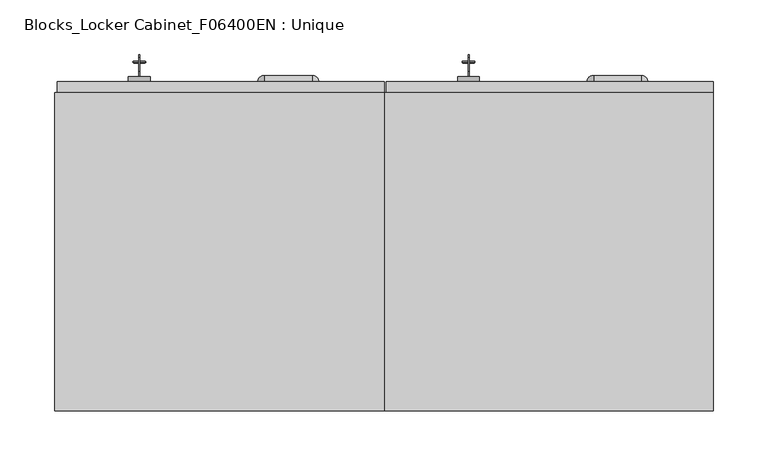
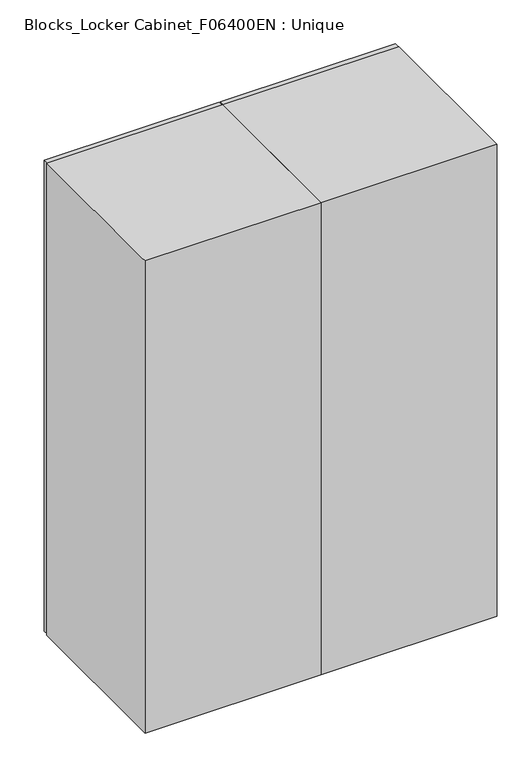
"""IFC4 building model written with IfcOpenShell, lengths in millimetres: furniture geometry, Blocks_Locker Cabinet_F06400EN : Unique."""

from ifc_helpers import new_model, si_unit, point, frame, frame_2d, origin, place, context, project, spatial, polyline, circle_curve, ellipse_curve, trimmed, segment, composite_curve, outline, extrude, faceted_brep, source, transform, mapped, element, save
from ifc_brep_helpers import plane_surface, cylinder_surface, revolved_surface, advanced_brep


def blocks_locker_cabinet_f06400en_unique_75e8493b(model_context):
    return source(origin(), model_context, "Body", "SolidModel", [
        advanced_brep(
        [(-83.0, 12.5, 1375.0), (-63.0, 12.5, 1375.0), (-71.1588195, 12.5, 1382.0962926), (-74.8411805, 12.5, 1382.0962926), (-74.8411805, 12.5, 1372.8618188), (-71.1588195, 12.5, 1372.8618188), (-83.0, 7.5, 1375.0), (-63.0, 7.5, 1375.0), (-63.0, 10.7450625, 1375.0), (-83.0, 10.7450625, 1375.0), (-71.1588195, 10.7450625, 1372.8618188), (-71.1588195, 10.7450625, 1382.0962926), (-74.8411805, 10.7450625, 1372.8618188), (-74.8411805, 10.7450625, 1382.0962926)],
        [
            (0, 1, circle_curve(frame((-73.0, 12.5, 1375.0), z_axis=(0.0, 1.0, 0.0), x_axis=(1.0, 0.0, 0.0)), 10.0)),
            (1, 0, circle_curve(frame((-73.0, 12.5, 1375.0), z_axis=(0.0, 1.0, 0.0), x_axis=(1.0, 0.0, 0.0)), 10.0)),
            (2, 3),
            (3, 4),
            (4, 5),
            (5, 2),
            (6, 7, circle_curve(frame((-73.0, 7.5, 1375.0), z_axis=(0.0, -1.0, 0.0), x_axis=(1.0, 0.0, 0.0)), 10.0)),
            (7, 6, circle_curve(frame((-73.0, 7.5, 1375.0), z_axis=(0.0, -1.0, 0.0), x_axis=(1.0, 0.0, 0.0)), 10.0)),
            (1, 8),
            (8, 7),
            (6, 9),
            (9, 0),
            (5, 10),
            (10, 11),
            (11, 2),
            (4, 12),
            (12, 10),
            (3, 13),
            (13, 12),
            (11, 13),
        ],
        [
            plane_surface(frame((-63.0, 12.5, 1375.0), z_axis=(0.0, 1.0, 0.0), x_axis=(0.0, 0.0, 1.0))),
            plane_surface(frame((-63.0, 7.5, 1375.0), z_axis=(0.0, -1.0, 0.0), x_axis=(0.0, 0.0, -1.0))),
            cylinder_surface(frame((-73.0, 7.5, 1375.0), z_axis=(0.0, 1.0, 0.0), x_axis=(1.0, 0.0, 0.0)), 10.0),
            plane_surface(frame((-71.1588195, 12.5, 1382.0962926), z_axis=(-1.0, 0.0, 0.0), x_axis=(0.0, -1.0, 0.0))),
            plane_surface(frame((-71.1588195, 12.5, 1372.8618188), z_axis=(0.0, 0.0, 1.0), x_axis=(0.0, -1.0, 0.0))),
            plane_surface(frame((-74.8411805, 12.5, 1372.8618188), z_axis=(1.0, 0.0, 0.0), x_axis=(0.0, -1.0, 0.0))),
            plane_surface(frame((-74.8411805, 12.5, 1382.0962926), z_axis=(0.0, 0.0, -1.0), x_axis=(0.0, -1.0, 0.0))),
            plane_surface(frame((-63.0, 10.7450625, 1375.0), z_axis=(0.0, 1.0, 0.0), x_axis=(0.0, 0.0, 1.0))),
        ],
        [
            (0, [[1, 2], [3, 4, 5, 6]]),
            (1, [[7, 8]]),
            (2, [[9, 10, -7, 11, 12, -2]]),
            (2, [[-12, -11, -8, -10, -9, -1]]),
            (3, [[13, 14, 15, -6]]),
            (4, [[16, 17, -13, -5]]),
            (5, [[18, 19, -16, -4]]),
            (6, [[-15, 20, -18, -3]]),
            (7, [[-17, -19, -20, -14]]),
        ],
    ),
        extrude(outline(composite_curve([segment(polyline([(16.8246351, 1372.8618188), (13.7848488, 1372.8618188)]), True, "CONTINUOUS"), segment(trimmed(circle_curve(frame_2d((12.908516, 1372.8618188)), 0.8763328), [point((13.7848488, 1372.8618188))], [point((12.0321832, 1372.8618188))], True, "CARTESIAN"), True, "CONTINUOUS"), segment(polyline([(12.0321832, 1372.8618188), (10.7450625, 1372.8618188), (10.7450625, 1377.6669902), (17.0336838, 1377.6669902)]), True, "CONTINUOUS"), segment(trimmed(circle_curve(frame_2d((23.0067332, 1375.0)), 6.5414185), [point((17.0336838, 1377.6669902))], [point((16.8246351, 1372.8618188))], False, "CARTESIAN"), True, "CONTINUOUS")], self_intersect=False), holes=[composite_curve([segment(trimmed(circle_curve(frame_2d((25.6281997, 1375.0)), 1.688217), [point((27.3164167, 1375.0))], [point((23.9399827, 1375.0))], True, "CARTESIAN"), True, "CONTINUOUS"), segment(trimmed(circle_curve(frame_2d((25.6281997, 1375.0)), 1.688217), [point((23.9399827, 1375.0))], [point((27.3164167, 1375.0))], True, "CARTESIAN"), True, "CONTINUOUS")], self_intersect=False)]), frame((-73.4043078, 0.0, 0.0), z_axis=(1.0, 0.0, 0.0), x_axis=(0.0, 1.0, 0.0)), (0.0, 0.0, 1.0), 0.9157402),
        extrude(outline(composite_curve([segment(polyline([(27.8125, 1354.8018875), (27.8125, 1351.7621012)]), True, "CONTINUOUS"), segment(trimmed(circle_curve(frame_2d((27.8125, 1350.8857684)), 0.8763328), [point((27.8125, 1351.7621012))], [point((27.8125, 1350.0094356))], True, "CARTESIAN"), True, "CONTINUOUS"), segment(polyline([(27.8125, 1350.0094356), (27.8125, 1347.7621012)]), True, "CONTINUOUS"), segment(trimmed(circle_curve(frame_2d((27.8125, 1346.8857684)), 0.8763328), [point((27.8125, 1347.7621012))], [point((27.8125, 1346.0094356))], True, "CARTESIAN"), True, "CONTINUOUS"), segment(polyline([(27.8125, 1346.0094356), (27.8125, 1343.7621012)]), True, "CONTINUOUS"), segment(trimmed(circle_curve(frame_2d((27.8125, 1342.8857684)), 0.8763328), [point((27.8125, 1343.7621012))], [point((27.8125, 1342.0094356))], True, "CARTESIAN"), True, "CONTINUOUS"), segment(polyline([(27.8125, 1342.0094356), (27.8125, 1340.3532579), (25.9613419, 1337.7095301), (24.2573286, 1337.7095301), (24.2573286, 1354.5978839)]), True, "CONTINUOUS"), segment(trimmed(circle_curve(frame_2d((25.6743188, 1360.9839856)), 6.5414185), [point((24.2573286, 1354.5978839))], [point((27.8125, 1354.8018875))], False, "CARTESIAN"), True, "CONTINUOUS")], self_intersect=False), holes=[composite_curve([segment(trimmed(circle_curve(frame_2d((25.6743188, 1363.6054521)), 1.688217), [point((25.6743188, 1365.2936691))], [point((25.6743188, 1361.9172351))], True, "CARTESIAN"), True, "CONTINUOUS"), segment(trimmed(circle_curve(frame_2d((25.6743188, 1363.6054521)), 1.688217), [point((25.6743188, 1361.9172351))], [point((25.6743188, 1365.2936691))], True, "CARTESIAN"), True, "CONTINUOUS")], self_intersect=False)]), frame((-73.4043078, 0.0, 0.0), z_axis=(1.0, 0.0, 0.0), x_axis=(0.0, 1.0, 0.0)), (0.0, 0.0, 1.0), 0.9157402),
        advanced_brep(
        [(-68.8, 25.663019, 1369.4000012), (-67.2, 25.663019, 1369.4000012), (-78.8, 25.663019, 1369.4000012), (-77.2, 25.663019, 1369.4000012)],
        [
            (0, 1, circle_curve(frame((-68.0, 25.663019, 1369.4000012), z_axis=(0.0, 0.0, -1.0), x_axis=(-1.0, 0.0, 0.0)), 0.8)),
            (1, 2, circle_curve(frame((-73.0, 25.663019, 1369.4000012), z_axis=(0.0, 1.0, 0.0), x_axis=(-1.0, 0.0, 0.0)), 5.8)),
            (2, 3, circle_curve(frame((-78.0, 25.663019, 1369.4000012), z_axis=(0.0, 0.0, -1.0), x_axis=(1.0, 0.0, 0.0)), 0.8)),
            (3, 0, circle_curve(frame((-73.0, 25.663019, 1369.4000012), z_axis=(0.0, -1.0, 0.0), x_axis=(-1.0, 0.0, 0.0)), 4.2)),
            (1, 0, circle_curve(frame((-68.0, 25.663019, 1369.4000012), z_axis=(0.0, 0.0, -1.0), x_axis=(-1.0, 0.0, 0.0)), 0.8)),
            (3, 2, circle_curve(frame((-78.0, 25.663019, 1369.4000012), z_axis=(0.0, 0.0, -1.0), x_axis=(1.0, 0.0, 0.0)), 0.8)),
            (2, 1, circle_curve(frame((-73.0, 25.663019, 1369.4000012), z_axis=(0.0, 1.0, 0.0), x_axis=(1.0, 0.0, 0.0)), 5.8)),
            (0, 3, circle_curve(frame((-73.0, 25.663019, 1369.4000012), z_axis=(0.0, -1.0, 0.0), x_axis=(1.0, 0.0, 0.0)), 4.2)),
        ],
        [
            revolved_surface(trimmed(ellipse_curve(frame((-78.0, 25.663019, 1369.4000012), z_axis=(0.0, 0.0, -1.0), x_axis=(1.0, 0.0, 0.0)), 0.8, 0.8), [point((-78.8, 25.663019, 1369.4000012))], [point((-77.2, 25.663019, 1369.4000012))], True, "CARTESIAN"), (-73.0, -2.5, 1369.4000012), (0.0, 1.0, 0.0)),
            revolved_surface(trimmed(ellipse_curve(frame((-78.0, 25.663019, 1369.4000012), z_axis=(0.0, 0.0, -1.0), x_axis=(1.0, 0.0, 0.0)), 0.8, 0.8), [point((-77.2, 25.663019, 1369.4000012))], [point((-78.8, 25.663019, 1369.4000012))], True, "CARTESIAN"), (-73.0, -2.5, 1369.4000012), (0.0, 1.0, 0.0)),
            revolved_surface(trimmed(ellipse_curve(frame((-68.0, 25.663019, 1369.4000012), z_axis=(0.0, 0.0, 1.0), x_axis=(-1.0, 0.0, 0.0)), 0.8, 0.8), [point((-67.2, 25.663019, 1369.4000012))], [point((-68.8, 25.663019, 1369.4000012))], True, "CARTESIAN"), (-73.0, -2.5, 1369.4000012), (0.0, 1.0, 0.0)),
            revolved_surface(trimmed(ellipse_curve(frame((-68.0, 25.663019, 1369.4000012), z_axis=(0.0, 0.0, 1.0), x_axis=(-1.0, 0.0, 0.0)), 0.8, 0.8), [point((-68.8, 25.663019, 1369.4000012))], [point((-67.2, 25.663019, 1369.4000012))], True, "CARTESIAN"), (-73.0, -2.5, 1369.4000012), (0.0, 1.0, 0.0)),
        ],
        [
            (0, [[1, 2, 3, 4]]),
            (1, [[5, -4, 6, -2]]),
            (2, [[-3, 7, -1, 8]]),
            (3, [[-6, -8, -5, -7]]),
        ],
    ),
        advanced_brep(
        [(-148.0, 7.5, 1799.0), (-148.0, -2.5, 1799.0), (150.0, -2.5, 1799.0), (150.0, 7.5, 1799.0), (-148.0, 7.5, 951.0), (150.0, 7.5, 951.0), (150.0, -2.5, 951.0), (-148.0, -2.5, 951.0), (-93.0, 7.5, 1525.0), (-93.0, 7.5, 1405.0), (-33.7890736, 7.5, 1405.0), (-33.7890736, 7.5, 1525.0), (-80.6526901, 0.3712773, 1525.0), (-57.2105549, 3.975278, 1525.0), (-80.6526901, 0.3712773, 1405.0), (-57.2105549, 3.975278, 1405.0)],
        [
            (0, 1),
            (1, 2),
            (2, 3),
            (3, 0),
            (4, 5),
            (5, 6),
            (6, 7),
            (7, 4),
            (3, 5),
            (4, 0),
            (8, 9),
            (9, 10),
            (10, 11),
            (11, 8),
            (2, 6),
            (1, 7),
            (12, 8),
            (11, 13),
            (13, 12, circle_curve(frame((-71.1776523, 16.7825242, 1525.0), z_axis=(0.0, 0.0, -1.0), x_axis=(0.0, 1.0, 0.0)), 18.9500756)),
            (14, 15, circle_curve(frame((-71.1776523, 16.7825242, 1405.0), z_axis=(0.0, 0.0, 1.0), x_axis=(0.0, 1.0, 0.0)), 18.9500756)),
            (15, 10),
            (9, 14),
            (12, 14),
            (15, 13),
        ],
        [
            plane_surface(frame((150.0, 7.5, 1799.0), z_axis=(0.0, 0.0, 1.0), x_axis=(1.0, 0.0, 0.0))),
            plane_surface(frame((150.0, 7.5, 951.0), z_axis=(0.0, 0.0, -1.0), x_axis=(-1.0, 0.0, 0.0))),
            plane_surface(frame((-148.0, 7.5, 1799.0), z_axis=(0.0, 1.0, 0.0), x_axis=(0.0, 0.0, -1.0))),
            plane_surface(frame((150.0, 7.5, 1799.0), z_axis=(1.0, 0.0, 0.0), x_axis=(0.0, 0.0, -1.0))),
            plane_surface(frame((150.0, -2.5, 1799.0), z_axis=(0.0, -1.0, 0.0), x_axis=(0.0, 0.0, -1.0))),
            plane_surface(frame((-148.0, -2.5, 1799.0), z_axis=(-1.0, 0.0, 0.0), x_axis=(0.0, 0.0, -1.0))),
            plane_surface(frame((-93.0, 7.5, 1525.0), z_axis=(0.0, 0.0, -1.0), x_axis=(-0.866025403784437, 0.5000000000000028, 0.0))),
            plane_surface(frame((-93.0, 7.5, 1405.0), z_axis=(0.0, 0.0, 1.0), x_axis=(0.866025403784437, -0.5000000000000028, 0.0))),
            plane_surface(frame((-80.6526901, 0.3712773, 1525.0), z_axis=(0.5000000000000028, 0.866025403784437, 0.0), x_axis=(0.0, 0.0, -1.0))),
            plane_surface(frame((-33.7890736, 7.5, 1525.0), z_axis=(-0.14881527984319862, 0.9888650122666847, 0.0), x_axis=(0.0, 0.0, -1.0))),
            revolved_surface(polyline([(-71.1776523, 35.7325998, 1525.0), (-71.1776523, 35.7325998, 1405.0)]), (-71.1776523, 16.7825242, 1405.0), (0.0, 0.0, 1.0)),
        ],
        [
            (0, [[1, 2, 3, 4]]),
            (1, [[5, 6, 7, 8]]),
            (2, [[9, -5, 10, -4], [11, 12, 13, 14]]),
            (3, [[15, -6, -9, -3]]),
            (4, [[16, -7, -15, -2]]),
            (5, [[-10, -8, -16, -1]]),
            (6, [[17, -14, 18, 19]]),
            (7, [[20, 21, -12, 22]]),
            (8, [[23, -22, -11, -17]]),
            (9, [[-13, -21, 24, -18]]),
            (10, [[-24, -20, -23, -19]]),
        ],
    ),
        advanced_brep(
        [(35.0, 7.5, 991.0), (90.5189667, 7.5, 991.0), (84.5189667, 7.5, 997.0), (41.0, 7.5, 997.0), (41.0, 13.5, 991.0), (84.5189667, 13.5, 991.0)],
        [
            (0, 1),
            (1, 2, circle_curve(frame((84.5189667, 7.5, 991.0), z_axis=(0.0, -1.0, 0.0), x_axis=(1.0, 0.0, 0.0)), 6.0)),
            (2, 3),
            (3, 0, circle_curve(frame((41.0, 7.5, 991.0), z_axis=(0.0, -1.0, 0.0), x_axis=(1.0, 0.0, 0.0)), 6.0)),
            (0, 4, circle_curve(frame((41.0, 7.5, 991.0), z_axis=(0.0, 0.0, -1.0), x_axis=(1.0, 0.0, 0.0)), 6.0)),
            (4, 5),
            (5, 1, circle_curve(frame((84.5189667, 7.5, 991.0), z_axis=(0.0, 0.0, -1.0), x_axis=(1.0, 0.0, 0.0)), 6.0)),
            (3, 4, circle_curve(frame((41.0, 7.5, 991.0), z_axis=(-1.0, 0.0, 0.0), x_axis=(0.0, 0.0, 1.0)), 6.0)),
            (2, 5, circle_curve(frame((84.5189667, 7.5, 991.0), z_axis=(-1.0, 0.0, 0.0), x_axis=(0.0, 0.0, 1.0)), 6.0)),
        ],
        [
            plane_surface(frame((85.0, 7.5, 991.0), z_axis=(0.0, -1.0, 0.0), x_axis=(0.0, 0.0, 1.0))),
            plane_surface(frame((85.0, 7.5, 991.0), z_axis=(0.0, 0.0, -1.0), x_axis=(0.0, 1.0, 0.0))),
            revolved_surface(trimmed(ellipse_curve(frame((41.0, 7.5, 991.0), z_axis=(0.0, 1.0, 0.0), x_axis=(1.0, 0.0, 0.0)), 6.0, 6.0), [point((35.0, 7.5, 991.0))], [point((41.0, 7.5, 997.0))], True, "CARTESIAN"), (85.0, 7.5, 991.0), (1.0, 0.0, 0.0)),
            cylinder_surface(frame((85.0, 7.5, 991.0), z_axis=(1.0, 0.0, 0.0), x_axis=(0.0, 0.0, 1.0)), 6.0),
            revolved_surface(trimmed(ellipse_curve(frame((84.5189667, 7.5, 991.0), z_axis=(0.0, 1.0, 0.0), x_axis=(1.0, 0.0, 0.0)), 6.0, 6.0), [point((84.5189667, 7.5, 997.0))], [point((90.5189667, 7.5, 991.0))], True, "CARTESIAN"), (85.0, 7.5, 991.0), (1.0, 0.0, 0.0)),
        ],
        [
            (0, [[1, 2, 3, 4]]),
            (1, [[-1, 5, 6, 7]]),
            (2, [[-5, -4, 8]]),
            (3, [[-6, -8, -3, 9]]),
            (4, [[-7, -9, -2]]),
        ],
    ),
        advanced_brep(
        [(35.0, 7.5, 1006.0), (90.5189667, 7.5, 1006.0), (84.5189667, 7.5, 1012.0), (41.0, 7.5, 1012.0), (41.0, 13.5, 1006.0), (84.5189667, 13.5, 1006.0)],
        [
            (0, 1),
            (1, 2, circle_curve(frame((84.5189667, 7.5, 1006.0), z_axis=(0.0, -1.0, 0.0), x_axis=(1.0, 0.0, 0.0)), 6.0)),
            (2, 3),
            (3, 0, circle_curve(frame((41.0, 7.5, 1006.0), z_axis=(0.0, -1.0, 0.0), x_axis=(1.0, 0.0, 0.0)), 6.0)),
            (0, 4, circle_curve(frame((41.0, 7.5, 1006.0), z_axis=(0.0, 0.0, -1.0), x_axis=(1.0, 0.0, 0.0)), 6.0)),
            (4, 5),
            (5, 1, circle_curve(frame((84.5189667, 7.5, 1006.0), z_axis=(0.0, 0.0, -1.0), x_axis=(1.0, 0.0, 0.0)), 6.0)),
            (3, 4, circle_curve(frame((41.0, 7.5, 1006.0), z_axis=(-1.0, 0.0, 0.0), x_axis=(0.0, 0.0, 1.0)), 6.0)),
            (2, 5, circle_curve(frame((84.5189667, 7.5, 1006.0), z_axis=(-1.0, 0.0, 0.0), x_axis=(0.0, 0.0, 1.0)), 6.0)),
        ],
        [
            plane_surface(frame((85.0, 7.5, 1006.0), z_axis=(0.0, -1.0, 0.0), x_axis=(0.0, 0.0, 1.0))),
            plane_surface(frame((85.0, 7.5, 1006.0), z_axis=(0.0, 0.0, -1.0), x_axis=(0.0, 1.0, 0.0))),
            revolved_surface(trimmed(ellipse_curve(frame((41.0, 7.5, 1006.0), z_axis=(0.0, 1.0, 0.0), x_axis=(1.0, 0.0, 0.0)), 6.0, 6.0), [point((35.0, 7.5, 1006.0))], [point((41.0, 7.5, 1012.0))], True, "CARTESIAN"), (85.0, 7.5, 1006.0), (1.0, 0.0, 0.0)),
            cylinder_surface(frame((85.0, 7.5, 1006.0), z_axis=(1.0, 0.0, 0.0), x_axis=(0.0, 0.0, 1.0)), 6.0),
            revolved_surface(trimmed(ellipse_curve(frame((84.5189667, 7.5, 1006.0), z_axis=(0.0, 1.0, 0.0), x_axis=(1.0, 0.0, 0.0)), 6.0, 6.0), [point((84.5189667, 7.5, 1012.0))], [point((90.5189667, 7.5, 1006.0))], True, "CARTESIAN"), (85.0, 7.5, 1006.0), (1.0, 0.0, 0.0)),
        ],
        [
            (0, [[1, 2, 3, 4]]),
            (1, [[-1, 5, 6, 7]]),
            (2, [[-5, -4, 8]]),
            (3, [[-6, -8, -3, 9]]),
            (4, [[-7, -9, -2]]),
        ],
    ),
        advanced_brep(
        [(35.0, 7.5, 1021.0), (90.5189667, 7.5, 1021.0), (84.5189667, 7.5, 1027.0), (41.0, 7.5, 1027.0), (41.0, 13.5, 1021.0), (84.5189667, 13.5, 1021.0)],
        [
            (0, 1),
            (1, 2, circle_curve(frame((84.5189667, 7.5, 1021.0), z_axis=(0.0, -1.0, 0.0), x_axis=(1.0, 0.0, 0.0)), 6.0)),
            (2, 3),
            (3, 0, circle_curve(frame((41.0, 7.5, 1021.0), z_axis=(0.0, -1.0, 0.0), x_axis=(1.0, 0.0, 0.0)), 6.0)),
            (0, 4, circle_curve(frame((41.0, 7.5, 1021.0), z_axis=(0.0, 0.0, -1.0), x_axis=(1.0, 0.0, 0.0)), 6.0)),
            (4, 5),
            (5, 1, circle_curve(frame((84.5189667, 7.5, 1021.0), z_axis=(0.0, 0.0, -1.0), x_axis=(1.0, 0.0, 0.0)), 6.0)),
            (3, 4, circle_curve(frame((41.0, 7.5, 1021.0), z_axis=(-1.0, 0.0, 0.0), x_axis=(0.0, 0.0, 1.0)), 6.0)),
            (2, 5, circle_curve(frame((84.5189667, 7.5, 1021.0), z_axis=(-1.0, 0.0, 0.0), x_axis=(0.0, 0.0, 1.0)), 6.0)),
        ],
        [
            plane_surface(frame((85.0, 7.5, 1021.0), z_axis=(0.0, -1.0, 0.0), x_axis=(0.0, 0.0, 1.0))),
            plane_surface(frame((85.0, 7.5, 1021.0), z_axis=(0.0, 0.0, -1.0), x_axis=(0.0, 1.0, 0.0))),
            revolved_surface(trimmed(ellipse_curve(frame((41.0, 7.5, 1021.0), z_axis=(0.0, 1.0, 0.0), x_axis=(1.0, 0.0, 0.0)), 6.0, 6.0), [point((35.0, 7.5, 1021.0))], [point((41.0, 7.5, 1027.0))], True, "CARTESIAN"), (85.0, 7.5, 1021.0), (1.0, 0.0, 0.0)),
            cylinder_surface(frame((85.0, 7.5, 1021.0), z_axis=(1.0, 0.0, 0.0), x_axis=(0.0, 0.0, 1.0)), 6.0),
            revolved_surface(trimmed(ellipse_curve(frame((84.5189667, 7.5, 1021.0), z_axis=(0.0, 1.0, 0.0), x_axis=(1.0, 0.0, 0.0)), 6.0, 6.0), [point((84.5189667, 7.5, 1027.0))], [point((90.5189667, 7.5, 1021.0))], True, "CARTESIAN"), (85.0, 7.5, 1021.0), (1.0, 0.0, 0.0)),
        ],
        [
            (0, [[1, 2, 3, 4]]),
            (1, [[-1, 5, 6, 7]]),
            (2, [[-5, -4, 8]]),
            (3, [[-6, -8, -3, 9]]),
            (4, [[-7, -9, -2]]),
        ],
    ),
        advanced_brep(
        [(35.0, 7.5, 1036.0), (90.5189667, 7.5, 1036.0), (84.5189667, 7.5, 1042.0), (41.0, 7.5, 1042.0), (41.0, 13.5, 1036.0), (84.5189667, 13.5, 1036.0)],
        [
            (0, 1),
            (1, 2, circle_curve(frame((84.5189667, 7.5, 1036.0), z_axis=(0.0, -1.0, 0.0), x_axis=(1.0, 0.0, 0.0)), 6.0)),
            (2, 3),
            (3, 0, circle_curve(frame((41.0, 7.5, 1036.0), z_axis=(0.0, -1.0, 0.0), x_axis=(1.0, 0.0, 0.0)), 6.0)),
            (0, 4, circle_curve(frame((41.0, 7.5, 1036.0), z_axis=(0.0, 0.0, -1.0), x_axis=(1.0, 0.0, 0.0)), 6.0)),
            (4, 5),
            (5, 1, circle_curve(frame((84.5189667, 7.5, 1036.0), z_axis=(0.0, 0.0, -1.0), x_axis=(1.0, 0.0, 0.0)), 6.0)),
            (3, 4, circle_curve(frame((41.0, 7.5, 1036.0), z_axis=(-1.0, 0.0, 0.0), x_axis=(0.0, 0.0, 1.0)), 6.0)),
            (2, 5, circle_curve(frame((84.5189667, 7.5, 1036.0), z_axis=(-1.0, 0.0, 0.0), x_axis=(0.0, 0.0, 1.0)), 6.0)),
        ],
        [
            plane_surface(frame((85.0, 7.5, 1036.0), z_axis=(0.0, -1.0, 0.0), x_axis=(0.0, 0.0, 1.0))),
            plane_surface(frame((85.0, 7.5, 1036.0), z_axis=(0.0, 0.0, -1.0), x_axis=(0.0, 1.0, 0.0))),
            revolved_surface(trimmed(ellipse_curve(frame((41.0, 7.5, 1036.0), z_axis=(0.0, 1.0, 0.0), x_axis=(1.0, 0.0, 0.0)), 6.0, 6.0), [point((35.0, 7.5, 1036.0))], [point((41.0, 7.5, 1042.0))], True, "CARTESIAN"), (85.0, 7.5, 1036.0), (1.0, 0.0, 0.0)),
            cylinder_surface(frame((85.0, 7.5, 1036.0), z_axis=(1.0, 0.0, 0.0), x_axis=(0.0, 0.0, 1.0)), 6.0),
            revolved_surface(trimmed(ellipse_curve(frame((84.5189667, 7.5, 1036.0), z_axis=(0.0, 1.0, 0.0), x_axis=(1.0, 0.0, 0.0)), 6.0, 6.0), [point((84.5189667, 7.5, 1042.0))], [point((90.5189667, 7.5, 1036.0))], True, "CARTESIAN"), (85.0, 7.5, 1036.0), (1.0, 0.0, 0.0)),
        ],
        [
            (0, [[1, 2, 3, 4]]),
            (1, [[-1, 5, 6, 7]]),
            (2, [[-5, -4, 8]]),
            (3, [[-6, -8, -3, 9]]),
            (4, [[-7, -9, -2]]),
        ],
    ),
        advanced_brep(
        [(35.0, 7.5, 1051.0), (90.5189667, 7.5, 1051.0), (84.5189667, 7.5, 1057.0), (41.0, 7.5, 1057.0), (41.0, 13.5, 1051.0), (84.5189667, 13.5, 1051.0)],
        [
            (0, 1),
            (1, 2, circle_curve(frame((84.5189667, 7.5, 1051.0), z_axis=(0.0, -1.0, 0.0), x_axis=(1.0, 0.0, 0.0)), 6.0)),
            (2, 3),
            (3, 0, circle_curve(frame((41.0, 7.5, 1051.0), z_axis=(0.0, -1.0, 0.0), x_axis=(1.0, 0.0, 0.0)), 6.0)),
            (0, 4, circle_curve(frame((41.0, 7.5, 1051.0), z_axis=(0.0, 0.0, -1.0), x_axis=(1.0, 0.0, 0.0)), 6.0)),
            (4, 5),
            (5, 1, circle_curve(frame((84.5189667, 7.5, 1051.0), z_axis=(0.0, 0.0, -1.0), x_axis=(1.0, 0.0, 0.0)), 6.0)),
            (3, 4, circle_curve(frame((41.0, 7.5, 1051.0), z_axis=(-1.0, 0.0, 0.0), x_axis=(0.0, 0.0, 1.0)), 6.0)),
            (2, 5, circle_curve(frame((84.5189667, 7.5, 1051.0), z_axis=(-1.0, 0.0, 0.0), x_axis=(0.0, 0.0, 1.0)), 6.0)),
        ],
        [
            plane_surface(frame((85.0, 7.5, 1051.0), z_axis=(0.0, -1.0, 0.0), x_axis=(0.0, 0.0, 1.0))),
            plane_surface(frame((85.0, 7.5, 1051.0), z_axis=(0.0, 0.0, -1.0), x_axis=(0.0, 1.0, 0.0))),
            revolved_surface(trimmed(ellipse_curve(frame((41.0, 7.5, 1051.0), z_axis=(0.0, 1.0, 0.0), x_axis=(1.0, 0.0, 0.0)), 6.0, 6.0), [point((35.0, 7.5, 1051.0))], [point((41.0, 7.5, 1057.0))], True, "CARTESIAN"), (85.0, 7.5, 1051.0), (1.0, 0.0, 0.0)),
            cylinder_surface(frame((85.0, 7.5, 1051.0), z_axis=(1.0, 0.0, 0.0), x_axis=(0.0, 0.0, 1.0)), 6.0),
            revolved_surface(trimmed(ellipse_curve(frame((84.5189667, 7.5, 1051.0), z_axis=(0.0, 1.0, 0.0), x_axis=(1.0, 0.0, 0.0)), 6.0, 6.0), [point((84.5189667, 7.5, 1057.0))], [point((90.5189667, 7.5, 1051.0))], True, "CARTESIAN"), (85.0, 7.5, 1051.0), (1.0, 0.0, 0.0)),
        ],
        [
            (0, [[1, 2, 3, 4]]),
            (1, [[-1, 5, 6, 7]]),
            (2, [[-5, -4, 8]]),
            (3, [[-6, -8, -3, 9]]),
            (4, [[-7, -9, -2]]),
        ],
    ),
        extrude(outline(composite_curve([segment(polyline([(-80.6526901, 0.3712773), (-93.0, 7.5), (-33.7890736, 7.5), (-57.2105549, 3.975278)]), True, "CONTINUOUS"), segment(trimmed(circle_curve(frame_2d((-71.1776523, 16.7825242)), 18.9500756), [point((-57.2105549, 3.975278))], [point((-80.6526901, 0.3712773))], False, "CARTESIAN"), True, "CONTINUOUS")], self_intersect=False)), frame((0.0, 0.0, 1405.0), z_axis=(0.0, 0.0, 1.0), x_axis=(1.0, 0.0, 0.0)), (0.0, 0.0, 1.0), 5.0),
        extrude(outline(composite_curve([segment(polyline([(-80.6526901, 0.3712773), (-93.0, 7.5), (-33.7890736, 7.5), (-57.2105549, 3.975278)]), True, "CONTINUOUS"), segment(trimmed(circle_curve(frame_2d((-71.1776523, 16.7825242)), 18.9500756), [point((-57.2105549, 3.975278))], [point((-80.6526901, 0.3712773))], False, "CARTESIAN"), True, "CONTINUOUS")], self_intersect=False)), frame((0.0, 0.0, 1520.0), z_axis=(0.0, 0.0, 1.0), x_axis=(1.0, 0.0, 0.0)), (0.0, 0.0, 1.0), 5.0),
        faceted_brep([(150.0, -2.5, 1800.0), (150.0, -2.5, 950.0), (-150.0, -2.5, 950.0), (-150.0, -2.5, 1800.0), (140.0, -2.5, 1790.0), (-140.0, -2.5, 1790.0), (-140.0, -2.5, 960.0), (140.0, -2.5, 960.0), (150.0, -292.5, 1800.0), (-150.0, -292.5, 1800.0), (-150.0, -292.5, 950.0), (150.0, -292.5, 950.0), (-150.0, -282.5, 1800.0), (150.0, -282.5, 1800.0), (-150.0, -282.5, 950.0), (150.0, -282.5, 950.0), (140.0, -282.5, 960.0), (140.0, -282.5, 1790.0), (-140.0, -282.5, 960.0), (-140.0, -282.5, 1790.0)], [[[0, 1, 2, 3], [4, 5, 6, 7]], [[8, 9, 10, 11]], [[3, 12, 9, 8, 13, 0]], [[2, 14, 10, 9, 12, 3]], [[1, 15, 11, 10, 14, 2]], [[0, 13, 8, 11, 15, 1]], [[7, 16, 17, 4]], [[6, 18, 16, 7]], [[5, 19, 18, 6]], [[4, 17, 19, 5]], [[16, 18, 19, 17]]]),
        advanced_brep(
        [(217.0, 12.5, 1375.0), (237.0, 12.5, 1375.0), (228.8411805, 12.5, 1382.0962926), (225.1588195, 12.5, 1382.0962926), (225.1588195, 12.5, 1372.8618188), (228.8411805, 12.5, 1372.8618188), (217.0, 7.5, 1375.0), (237.0, 7.5, 1375.0), (237.0, 10.7450625, 1375.0), (217.0, 10.7450625, 1375.0), (228.8411805, 10.7450625, 1372.8618188), (228.8411805, 10.7450625, 1382.0962926), (225.1588195, 10.7450625, 1372.8618188), (225.1588195, 10.7450625, 1382.0962926)],
        [
            (0, 1, circle_curve(frame((227.0, 12.5, 1375.0), z_axis=(0.0, 1.0, 0.0), x_axis=(1.0, 0.0, 0.0)), 10.0)),
            (1, 0, circle_curve(frame((227.0, 12.5, 1375.0), z_axis=(0.0, 1.0, 0.0), x_axis=(1.0, 0.0, 0.0)), 10.0)),
            (2, 3),
            (3, 4),
            (4, 5),
            (5, 2),
            (6, 7, circle_curve(frame((227.0, 7.5, 1375.0), z_axis=(0.0, -1.0, 0.0), x_axis=(1.0, 0.0, 0.0)), 10.0)),
            (7, 6, circle_curve(frame((227.0, 7.5, 1375.0), z_axis=(0.0, -1.0, 0.0), x_axis=(1.0, 0.0, 0.0)), 10.0)),
            (1, 8),
            (8, 7),
            (6, 9),
            (9, 0),
            (5, 10),
            (10, 11),
            (11, 2),
            (4, 12),
            (12, 10),
            (3, 13),
            (13, 12),
            (11, 13),
        ],
        [
            plane_surface(frame((237.0, 12.5, 1375.0), z_axis=(0.0, 1.0, 0.0), x_axis=(0.0, 0.0, 1.0))),
            plane_surface(frame((237.0, 7.5, 1375.0), z_axis=(0.0, -1.0, 0.0), x_axis=(0.0, 0.0, -1.0))),
            cylinder_surface(frame((227.0, 7.5, 1375.0), z_axis=(0.0, 1.0, 0.0), x_axis=(1.0, 0.0, 0.0)), 10.0),
            plane_surface(frame((228.8411805, 12.5, 1382.0962926), z_axis=(-1.0, 0.0, 0.0), x_axis=(0.0, -1.0, 0.0))),
            plane_surface(frame((228.8411805, 12.5, 1372.8618188), z_axis=(0.0, 0.0, 1.0), x_axis=(0.0, -1.0, 0.0))),
            plane_surface(frame((225.1588195, 12.5, 1372.8618188), z_axis=(1.0, 0.0, 0.0), x_axis=(0.0, -1.0, 0.0))),
            plane_surface(frame((225.1588195, 12.5, 1382.0962926), z_axis=(0.0, 0.0, -1.0), x_axis=(0.0, -1.0, 0.0))),
            plane_surface(frame((237.0, 10.7450625, 1375.0), z_axis=(0.0, 1.0, 0.0), x_axis=(0.0, 0.0, 1.0))),
        ],
        [
            (0, [[1, 2], [3, 4, 5, 6]]),
            (1, [[7, 8]]),
            (2, [[9, 10, -7, 11, 12, -2]]),
            (2, [[-12, -11, -8, -10, -9, -1]]),
            (3, [[13, 14, 15, -6]]),
            (4, [[16, 17, -13, -5]]),
            (5, [[18, 19, -16, -4]]),
            (6, [[-15, 20, -18, -3]]),
            (7, [[-17, -19, -20, -14]]),
        ],
    ),
        extrude(outline(composite_curve([segment(polyline([(16.8246351, 1372.8618188), (13.7848488, 1372.8618188)]), True, "CONTINUOUS"), segment(trimmed(circle_curve(frame_2d((12.908516, 1372.8618188)), 0.8763328), [point((13.7848488, 1372.8618188))], [point((12.0321832, 1372.8618188))], True, "CARTESIAN"), True, "CONTINUOUS"), segment(polyline([(12.0321832, 1372.8618188), (10.7450625, 1372.8618188), (10.7450625, 1377.6669902), (17.0336838, 1377.6669902)]), True, "CONTINUOUS"), segment(trimmed(circle_curve(frame_2d((23.0067332, 1375.0)), 6.5414185), [point((17.0336838, 1377.6669902))], [point((16.8246351, 1372.8618188))], False, "CARTESIAN"), True, "CONTINUOUS")], self_intersect=False), holes=[composite_curve([segment(trimmed(circle_curve(frame_2d((25.6281997, 1375.0)), 1.688217), [point((27.3164167, 1375.0))], [point((23.9399827, 1375.0))], True, "CARTESIAN"), True, "CONTINUOUS"), segment(trimmed(circle_curve(frame_2d((25.6281997, 1375.0)), 1.688217), [point((23.9399827, 1375.0))], [point((27.3164167, 1375.0))], True, "CARTESIAN"), True, "CONTINUOUS")], self_intersect=False)]), frame((226.5956922, 0.0, 0.0), z_axis=(1.0, 0.0, 0.0), x_axis=(0.0, 1.0, 0.0)), (0.0, 0.0, 1.0), 0.9157402),
        extrude(outline(composite_curve([segment(polyline([(27.8125, 1354.8018875), (27.8125, 1351.7621012)]), True, "CONTINUOUS"), segment(trimmed(circle_curve(frame_2d((27.8125, 1350.8857684)), 0.8763328), [point((27.8125, 1351.7621012))], [point((27.8125, 1350.0094356))], True, "CARTESIAN"), True, "CONTINUOUS"), segment(polyline([(27.8125, 1350.0094356), (27.8125, 1347.7621012)]), True, "CONTINUOUS"), segment(trimmed(circle_curve(frame_2d((27.8125, 1346.8857684)), 0.8763328), [point((27.8125, 1347.7621012))], [point((27.8125, 1346.0094356))], True, "CARTESIAN"), True, "CONTINUOUS"), segment(polyline([(27.8125, 1346.0094356), (27.8125, 1343.7621012)]), True, "CONTINUOUS"), segment(trimmed(circle_curve(frame_2d((27.8125, 1342.8857684)), 0.8763328), [point((27.8125, 1343.7621012))], [point((27.8125, 1342.0094356))], True, "CARTESIAN"), True, "CONTINUOUS"), segment(polyline([(27.8125, 1342.0094356), (27.8125, 1340.3532579), (25.9613419, 1337.7095301), (24.2573286, 1337.7095301), (24.2573286, 1354.5978839)]), True, "CONTINUOUS"), segment(trimmed(circle_curve(frame_2d((25.6743188, 1360.9839856)), 6.5414185), [point((24.2573286, 1354.5978839))], [point((27.8125, 1354.8018875))], False, "CARTESIAN"), True, "CONTINUOUS")], self_intersect=False), holes=[composite_curve([segment(trimmed(circle_curve(frame_2d((25.6743188, 1363.6054521)), 1.688217), [point((25.6743188, 1365.2936691))], [point((25.6743188, 1361.9172351))], True, "CARTESIAN"), True, "CONTINUOUS"), segment(trimmed(circle_curve(frame_2d((25.6743188, 1363.6054521)), 1.688217), [point((25.6743188, 1361.9172351))], [point((25.6743188, 1365.2936691))], True, "CARTESIAN"), True, "CONTINUOUS")], self_intersect=False)]), frame((226.5956922, 0.0, 0.0), z_axis=(1.0, 0.0, 0.0), x_axis=(0.0, 1.0, 0.0)), (0.0, 0.0, 1.0), 0.9157402),
        advanced_brep(
        [(231.2, 25.663019, 1369.4000012), (232.8, 25.663019, 1369.4000012), (221.2, 25.663019, 1369.4000012), (222.8, 25.663019, 1369.4000012)],
        [
            (0, 1, circle_curve(frame((232.0, 25.663019, 1369.4000012), z_axis=(0.0, 0.0, -1.0), x_axis=(-1.0, 0.0, 0.0)), 0.8)),
            (1, 2, circle_curve(frame((227.0, 25.663019, 1369.4000012), z_axis=(0.0, 1.0, 0.0), x_axis=(-1.0, 0.0, 0.0)), 5.8)),
            (2, 3, circle_curve(frame((222.0, 25.663019, 1369.4000012), z_axis=(0.0, 0.0, -1.0), x_axis=(1.0, 0.0, 0.0)), 0.8)),
            (3, 0, circle_curve(frame((227.0, 25.663019, 1369.4000012), z_axis=(0.0, -1.0, 0.0), x_axis=(-1.0, 0.0, 0.0)), 4.2)),
            (1, 0, circle_curve(frame((232.0, 25.663019, 1369.4000012), z_axis=(0.0, 0.0, -1.0), x_axis=(-1.0, 0.0, 0.0)), 0.8)),
            (3, 2, circle_curve(frame((222.0, 25.663019, 1369.4000012), z_axis=(0.0, 0.0, -1.0), x_axis=(1.0, 0.0, 0.0)), 0.8)),
            (2, 1, circle_curve(frame((227.0, 25.663019, 1369.4000012), z_axis=(0.0, 1.0, 0.0), x_axis=(1.0, 0.0, 0.0)), 5.8)),
            (0, 3, circle_curve(frame((227.0, 25.663019, 1369.4000012), z_axis=(0.0, -1.0, 0.0), x_axis=(1.0, 0.0, 0.0)), 4.2)),
        ],
        [
            revolved_surface(trimmed(ellipse_curve(frame((222.0, 25.663019, 1369.4000012), z_axis=(0.0, 0.0, -1.0), x_axis=(1.0, 0.0, 0.0)), 0.8, 0.8), [point((221.2, 25.663019, 1369.4000012))], [point((222.8, 25.663019, 1369.4000012))], True, "CARTESIAN"), (227.0, -2.5, 1369.4000012), (0.0, 1.0, 0.0)),
            revolved_surface(trimmed(ellipse_curve(frame((222.0, 25.663019, 1369.4000012), z_axis=(0.0, 0.0, -1.0), x_axis=(1.0, 0.0, 0.0)), 0.8, 0.8), [point((222.8, 25.663019, 1369.4000012))], [point((221.2, 25.663019, 1369.4000012))], True, "CARTESIAN"), (227.0, -2.5, 1369.4000012), (0.0, 1.0, 0.0)),
            revolved_surface(trimmed(ellipse_curve(frame((232.0, 25.663019, 1369.4000012), z_axis=(0.0, 0.0, 1.0), x_axis=(-1.0, 0.0, 0.0)), 0.8, 0.8), [point((232.8, 25.663019, 1369.4000012))], [point((231.2, 25.663019, 1369.4000012))], True, "CARTESIAN"), (227.0, -2.5, 1369.4000012), (0.0, 1.0, 0.0)),
            revolved_surface(trimmed(ellipse_curve(frame((232.0, 25.663019, 1369.4000012), z_axis=(0.0, 0.0, 1.0), x_axis=(-1.0, 0.0, 0.0)), 0.8, 0.8), [point((231.2, 25.663019, 1369.4000012))], [point((232.8, 25.663019, 1369.4000012))], True, "CARTESIAN"), (227.0, -2.5, 1369.4000012), (0.0, 1.0, 0.0)),
        ],
        [
            (0, [[1, 2, 3, 4]]),
            (1, [[5, -4, 6, -2]]),
            (2, [[-3, 7, -1, 8]]),
            (3, [[-6, -8, -5, -7]]),
        ],
    ),
        advanced_brep(
        [(152.0, 7.5, 1799.0), (152.0, -2.5, 1799.0), (450.0, -2.5, 1799.0), (450.0, 7.5, 1799.0), (152.0, 7.5, 951.0), (450.0, 7.5, 951.0), (450.0, -2.5, 951.0), (152.0, -2.5, 951.0), (207.0, 7.5, 1525.0), (207.0, 7.5, 1405.0), (266.2109264, 7.5, 1405.0), (266.2109264, 7.5, 1525.0), (219.3473099, 0.3712773, 1525.0), (242.7894451, 3.975278, 1525.0), (219.3473099, 0.3712773, 1405.0), (242.7894451, 3.975278, 1405.0)],
        [
            (0, 1),
            (1, 2),
            (2, 3),
            (3, 0),
            (4, 5),
            (5, 6),
            (6, 7),
            (7, 4),
            (3, 5),
            (4, 0),
            (8, 9),
            (9, 10),
            (10, 11),
            (11, 8),
            (2, 6),
            (1, 7),
            (12, 8),
            (11, 13),
            (13, 12, circle_curve(frame((228.8223477, 16.7825242, 1525.0), z_axis=(0.0, 0.0, -1.0), x_axis=(0.0, 1.0, 0.0)), 18.9500756)),
            (14, 15, circle_curve(frame((228.8223477, 16.7825242, 1405.0), z_axis=(0.0, 0.0, 1.0), x_axis=(0.0, 1.0, 0.0)), 18.9500756)),
            (15, 10),
            (9, 14),
            (12, 14),
            (15, 13),
        ],
        [
            plane_surface(frame((450.0, 7.5, 1799.0), z_axis=(0.0, 0.0, 1.0), x_axis=(1.0, 0.0, 0.0))),
            plane_surface(frame((450.0, 7.5, 951.0), z_axis=(0.0, 0.0, -1.0), x_axis=(-1.0, 0.0, 0.0))),
            plane_surface(frame((152.0, 7.5, 1799.0), z_axis=(0.0, 1.0, 0.0), x_axis=(0.0, 0.0, -1.0))),
            plane_surface(frame((450.0, 7.5, 1799.0), z_axis=(1.0, 0.0, 0.0), x_axis=(0.0, 0.0, -1.0))),
            plane_surface(frame((450.0, -2.5, 1799.0), z_axis=(0.0, -1.0, 0.0), x_axis=(0.0, 0.0, -1.0))),
            plane_surface(frame((152.0, -2.5, 1799.0), z_axis=(-1.0, 0.0, 0.0), x_axis=(0.0, 0.0, -1.0))),
            plane_surface(frame((207.0, 7.5, 1525.0), z_axis=(0.0, 0.0, -1.0), x_axis=(-0.866025403784437, 0.5000000000000028, 0.0))),
            plane_surface(frame((207.0, 7.5, 1405.0), z_axis=(0.0, 0.0, 1.0), x_axis=(0.866025403784437, -0.5000000000000028, 0.0))),
            plane_surface(frame((219.3473099, 0.3712773, 1525.0), z_axis=(0.5000000000000028, 0.866025403784437, 0.0), x_axis=(0.0, 0.0, -1.0))),
            plane_surface(frame((266.2109264, 7.5, 1525.0), z_axis=(-0.14881527984319862, 0.9888650122666847, 0.0), x_axis=(0.0, 0.0, -1.0))),
            revolved_surface(polyline([(228.8223477, 35.7325998, 1525.0), (228.8223477, 35.7325998, 1405.0)]), (228.8223477, 16.7825242, 1405.0), (0.0, 0.0, 1.0)),
        ],
        [
            (0, [[1, 2, 3, 4]]),
            (1, [[5, 6, 7, 8]]),
            (2, [[9, -5, 10, -4], [11, 12, 13, 14]]),
            (3, [[15, -6, -9, -3]]),
            (4, [[16, -7, -15, -2]]),
            (5, [[-10, -8, -16, -1]]),
            (6, [[17, -14, 18, 19]]),
            (7, [[20, 21, -12, 22]]),
            (8, [[23, -22, -11, -17]]),
            (9, [[-13, -21, 24, -18]]),
            (10, [[-24, -20, -23, -19]]),
        ],
    ),
        advanced_brep(
        [(335.0, 7.5, 991.0), (390.5189667, 7.5, 991.0), (384.5189667, 7.5, 997.0), (341.0, 7.5, 997.0), (341.0, 13.5, 991.0), (384.5189667, 13.5, 991.0)],
        [
            (0, 1),
            (1, 2, circle_curve(frame((384.5189667, 7.5, 991.0), z_axis=(0.0, -1.0, 0.0), x_axis=(1.0, 0.0, 0.0)), 6.0)),
            (2, 3),
            (3, 0, circle_curve(frame((341.0, 7.5, 991.0), z_axis=(0.0, -1.0, 0.0), x_axis=(1.0, 0.0, 0.0)), 6.0)),
            (0, 4, circle_curve(frame((341.0, 7.5, 991.0), z_axis=(0.0, 0.0, -1.0), x_axis=(1.0, 0.0, 0.0)), 6.0)),
            (4, 5),
            (5, 1, circle_curve(frame((384.5189667, 7.5, 991.0), z_axis=(0.0, 0.0, -1.0), x_axis=(1.0, 0.0, 0.0)), 6.0)),
            (3, 4, circle_curve(frame((341.0, 7.5, 991.0), z_axis=(-1.0, 0.0, 0.0), x_axis=(0.0, 0.0, 1.0)), 6.0)),
            (2, 5, circle_curve(frame((384.5189667, 7.5, 991.0), z_axis=(-1.0, 0.0, 0.0), x_axis=(0.0, 0.0, 1.0)), 6.0)),
        ],
        [
            plane_surface(frame((385.0, 7.5, 991.0), z_axis=(0.0, -1.0, 0.0), x_axis=(0.0, 0.0, 1.0))),
            plane_surface(frame((385.0, 7.5, 991.0), z_axis=(0.0, 0.0, -1.0), x_axis=(0.0, 1.0, 0.0))),
            revolved_surface(trimmed(ellipse_curve(frame((341.0, 7.5, 991.0), z_axis=(0.0, 1.0, 0.0), x_axis=(1.0, 0.0, 0.0)), 6.0, 6.0), [point((335.0, 7.5, 991.0))], [point((341.0, 7.5, 997.0))], True, "CARTESIAN"), (385.0, 7.5, 991.0), (1.0, 0.0, 0.0)),
            cylinder_surface(frame((385.0, 7.5, 991.0), z_axis=(1.0, 0.0, 0.0), x_axis=(0.0, 0.0, 1.0)), 6.0),
            revolved_surface(trimmed(ellipse_curve(frame((384.5189667, 7.5, 991.0), z_axis=(0.0, 1.0, 0.0), x_axis=(1.0, 0.0, 0.0)), 6.0, 6.0), [point((384.5189667, 7.5, 997.0))], [point((390.5189667, 7.5, 991.0))], True, "CARTESIAN"), (385.0, 7.5, 991.0), (1.0, 0.0, 0.0)),
        ],
        [
            (0, [[1, 2, 3, 4]]),
            (1, [[-1, 5, 6, 7]]),
            (2, [[-5, -4, 8]]),
            (3, [[-6, -8, -3, 9]]),
            (4, [[-7, -9, -2]]),
        ],
    ),
        advanced_brep(
        [(335.0, 7.5, 1006.0), (390.5189667, 7.5, 1006.0), (384.5189667, 7.5, 1012.0), (341.0, 7.5, 1012.0), (341.0, 13.5, 1006.0), (384.5189667, 13.5, 1006.0)],
        [
            (0, 1),
            (1, 2, circle_curve(frame((384.5189667, 7.5, 1006.0), z_axis=(0.0, -1.0, 0.0), x_axis=(1.0, 0.0, 0.0)), 6.0)),
            (2, 3),
            (3, 0, circle_curve(frame((341.0, 7.5, 1006.0), z_axis=(0.0, -1.0, 0.0), x_axis=(1.0, 0.0, 0.0)), 6.0)),
            (0, 4, circle_curve(frame((341.0, 7.5, 1006.0), z_axis=(0.0, 0.0, -1.0), x_axis=(1.0, 0.0, 0.0)), 6.0)),
            (4, 5),
            (5, 1, circle_curve(frame((384.5189667, 7.5, 1006.0), z_axis=(0.0, 0.0, -1.0), x_axis=(1.0, 0.0, 0.0)), 6.0)),
            (3, 4, circle_curve(frame((341.0, 7.5, 1006.0), z_axis=(-1.0, 0.0, 0.0), x_axis=(0.0, 0.0, 1.0)), 6.0)),
            (2, 5, circle_curve(frame((384.5189667, 7.5, 1006.0), z_axis=(-1.0, 0.0, 0.0), x_axis=(0.0, 0.0, 1.0)), 6.0)),
        ],
        [
            plane_surface(frame((385.0, 7.5, 1006.0), z_axis=(0.0, -1.0, 0.0), x_axis=(0.0, 0.0, 1.0))),
            plane_surface(frame((385.0, 7.5, 1006.0), z_axis=(0.0, 0.0, -1.0), x_axis=(0.0, 1.0, 0.0))),
            revolved_surface(trimmed(ellipse_curve(frame((341.0, 7.5, 1006.0), z_axis=(0.0, 1.0, 0.0), x_axis=(1.0, 0.0, 0.0)), 6.0, 6.0), [point((335.0, 7.5, 1006.0))], [point((341.0, 7.5, 1012.0))], True, "CARTESIAN"), (385.0, 7.5, 1006.0), (1.0, 0.0, 0.0)),
            cylinder_surface(frame((385.0, 7.5, 1006.0), z_axis=(1.0, 0.0, 0.0), x_axis=(0.0, 0.0, 1.0)), 6.0),
            revolved_surface(trimmed(ellipse_curve(frame((384.5189667, 7.5, 1006.0), z_axis=(0.0, 1.0, 0.0), x_axis=(1.0, 0.0, 0.0)), 6.0, 6.0), [point((384.5189667, 7.5, 1012.0))], [point((390.5189667, 7.5, 1006.0))], True, "CARTESIAN"), (385.0, 7.5, 1006.0), (1.0, 0.0, 0.0)),
        ],
        [
            (0, [[1, 2, 3, 4]]),
            (1, [[-1, 5, 6, 7]]),
            (2, [[-5, -4, 8]]),
            (3, [[-6, -8, -3, 9]]),
            (4, [[-7, -9, -2]]),
        ],
    ),
        advanced_brep(
        [(335.0, 7.5, 1021.0), (390.5189667, 7.5, 1021.0), (384.5189667, 7.5, 1027.0), (341.0, 7.5, 1027.0), (341.0, 13.5, 1021.0), (384.5189667, 13.5, 1021.0)],
        [
            (0, 1),
            (1, 2, circle_curve(frame((384.5189667, 7.5, 1021.0), z_axis=(0.0, -1.0, 0.0), x_axis=(1.0, 0.0, 0.0)), 6.0)),
            (2, 3),
            (3, 0, circle_curve(frame((341.0, 7.5, 1021.0), z_axis=(0.0, -1.0, 0.0), x_axis=(1.0, 0.0, 0.0)), 6.0)),
            (0, 4, circle_curve(frame((341.0, 7.5, 1021.0), z_axis=(0.0, 0.0, -1.0), x_axis=(1.0, 0.0, 0.0)), 6.0)),
            (4, 5),
            (5, 1, circle_curve(frame((384.5189667, 7.5, 1021.0), z_axis=(0.0, 0.0, -1.0), x_axis=(1.0, 0.0, 0.0)), 6.0)),
            (3, 4, circle_curve(frame((341.0, 7.5, 1021.0), z_axis=(-1.0, 0.0, 0.0), x_axis=(0.0, 0.0, 1.0)), 6.0)),
            (2, 5, circle_curve(frame((384.5189667, 7.5, 1021.0), z_axis=(-1.0, 0.0, 0.0), x_axis=(0.0, 0.0, 1.0)), 6.0)),
        ],
        [
            plane_surface(frame((385.0, 7.5, 1021.0), z_axis=(0.0, -1.0, 0.0), x_axis=(0.0, 0.0, 1.0))),
            plane_surface(frame((385.0, 7.5, 1021.0), z_axis=(0.0, 0.0, -1.0), x_axis=(0.0, 1.0, 0.0))),
            revolved_surface(trimmed(ellipse_curve(frame((341.0, 7.5, 1021.0), z_axis=(0.0, 1.0, 0.0), x_axis=(1.0, 0.0, 0.0)), 6.0, 6.0), [point((335.0, 7.5, 1021.0))], [point((341.0, 7.5, 1027.0))], True, "CARTESIAN"), (385.0, 7.5, 1021.0), (1.0, 0.0, 0.0)),
            cylinder_surface(frame((385.0, 7.5, 1021.0), z_axis=(1.0, 0.0, 0.0), x_axis=(0.0, 0.0, 1.0)), 6.0),
            revolved_surface(trimmed(ellipse_curve(frame((384.5189667, 7.5, 1021.0), z_axis=(0.0, 1.0, 0.0), x_axis=(1.0, 0.0, 0.0)), 6.0, 6.0), [point((384.5189667, 7.5, 1027.0))], [point((390.5189667, 7.5, 1021.0))], True, "CARTESIAN"), (385.0, 7.5, 1021.0), (1.0, 0.0, 0.0)),
        ],
        [
            (0, [[1, 2, 3, 4]]),
            (1, [[-1, 5, 6, 7]]),
            (2, [[-5, -4, 8]]),
            (3, [[-6, -8, -3, 9]]),
            (4, [[-7, -9, -2]]),
        ],
    ),
        advanced_brep(
        [(335.0, 7.5, 1036.0), (390.5189667, 7.5, 1036.0), (384.5189667, 7.5, 1042.0), (341.0, 7.5, 1042.0), (341.0, 13.5, 1036.0), (384.5189667, 13.5, 1036.0)],
        [
            (0, 1),
            (1, 2, circle_curve(frame((384.5189667, 7.5, 1036.0), z_axis=(0.0, -1.0, 0.0), x_axis=(1.0, 0.0, 0.0)), 6.0)),
            (2, 3),
            (3, 0, circle_curve(frame((341.0, 7.5, 1036.0), z_axis=(0.0, -1.0, 0.0), x_axis=(1.0, 0.0, 0.0)), 6.0)),
            (0, 4, circle_curve(frame((341.0, 7.5, 1036.0), z_axis=(0.0, 0.0, -1.0), x_axis=(1.0, 0.0, 0.0)), 6.0)),
            (4, 5),
            (5, 1, circle_curve(frame((384.5189667, 7.5, 1036.0), z_axis=(0.0, 0.0, -1.0), x_axis=(1.0, 0.0, 0.0)), 6.0)),
            (3, 4, circle_curve(frame((341.0, 7.5, 1036.0), z_axis=(-1.0, 0.0, 0.0), x_axis=(0.0, 0.0, 1.0)), 6.0)),
            (2, 5, circle_curve(frame((384.5189667, 7.5, 1036.0), z_axis=(-1.0, 0.0, 0.0), x_axis=(0.0, 0.0, 1.0)), 6.0)),
        ],
        [
            plane_surface(frame((385.0, 7.5, 1036.0), z_axis=(0.0, -1.0, 0.0), x_axis=(0.0, 0.0, 1.0))),
            plane_surface(frame((385.0, 7.5, 1036.0), z_axis=(0.0, 0.0, -1.0), x_axis=(0.0, 1.0, 0.0))),
            revolved_surface(trimmed(ellipse_curve(frame((341.0, 7.5, 1036.0), z_axis=(0.0, 1.0, 0.0), x_axis=(1.0, 0.0, 0.0)), 6.0, 6.0), [point((335.0, 7.5, 1036.0))], [point((341.0, 7.5, 1042.0))], True, "CARTESIAN"), (385.0, 7.5, 1036.0), (1.0, 0.0, 0.0)),
            cylinder_surface(frame((385.0, 7.5, 1036.0), z_axis=(1.0, 0.0, 0.0), x_axis=(0.0, 0.0, 1.0)), 6.0),
            revolved_surface(trimmed(ellipse_curve(frame((384.5189667, 7.5, 1036.0), z_axis=(0.0, 1.0, 0.0), x_axis=(1.0, 0.0, 0.0)), 6.0, 6.0), [point((384.5189667, 7.5, 1042.0))], [point((390.5189667, 7.5, 1036.0))], True, "CARTESIAN"), (385.0, 7.5, 1036.0), (1.0, 0.0, 0.0)),
        ],
        [
            (0, [[1, 2, 3, 4]]),
            (1, [[-1, 5, 6, 7]]),
            (2, [[-5, -4, 8]]),
            (3, [[-6, -8, -3, 9]]),
            (4, [[-7, -9, -2]]),
        ],
    ),
        advanced_brep(
        [(335.0, 7.5, 1051.0), (390.5189667, 7.5, 1051.0), (384.5189667, 7.5, 1057.0), (341.0, 7.5, 1057.0), (341.0, 13.5, 1051.0), (384.5189667, 13.5, 1051.0)],
        [
            (0, 1),
            (1, 2, circle_curve(frame((384.5189667, 7.5, 1051.0), z_axis=(0.0, -1.0, 0.0), x_axis=(1.0, 0.0, 0.0)), 6.0)),
            (2, 3),
            (3, 0, circle_curve(frame((341.0, 7.5, 1051.0), z_axis=(0.0, -1.0, 0.0), x_axis=(1.0, 0.0, 0.0)), 6.0)),
            (0, 4, circle_curve(frame((341.0, 7.5, 1051.0), z_axis=(0.0, 0.0, -1.0), x_axis=(1.0, 0.0, 0.0)), 6.0)),
            (4, 5),
            (5, 1, circle_curve(frame((384.5189667, 7.5, 1051.0), z_axis=(0.0, 0.0, -1.0), x_axis=(1.0, 0.0, 0.0)), 6.0)),
            (3, 4, circle_curve(frame((341.0, 7.5, 1051.0), z_axis=(-1.0, 0.0, 0.0), x_axis=(0.0, 0.0, 1.0)), 6.0)),
            (2, 5, circle_curve(frame((384.5189667, 7.5, 1051.0), z_axis=(-1.0, 0.0, 0.0), x_axis=(0.0, 0.0, 1.0)), 6.0)),
        ],
        [
            plane_surface(frame((385.0, 7.5, 1051.0), z_axis=(0.0, -1.0, 0.0), x_axis=(0.0, 0.0, 1.0))),
            plane_surface(frame((385.0, 7.5, 1051.0), z_axis=(0.0, 0.0, -1.0), x_axis=(0.0, 1.0, 0.0))),
            revolved_surface(trimmed(ellipse_curve(frame((341.0, 7.5, 1051.0), z_axis=(0.0, 1.0, 0.0), x_axis=(1.0, 0.0, 0.0)), 6.0, 6.0), [point((335.0, 7.5, 1051.0))], [point((341.0, 7.5, 1057.0))], True, "CARTESIAN"), (385.0, 7.5, 1051.0), (1.0, 0.0, 0.0)),
            cylinder_surface(frame((385.0, 7.5, 1051.0), z_axis=(1.0, 0.0, 0.0), x_axis=(0.0, 0.0, 1.0)), 6.0),
            revolved_surface(trimmed(ellipse_curve(frame((384.5189667, 7.5, 1051.0), z_axis=(0.0, 1.0, 0.0), x_axis=(1.0, 0.0, 0.0)), 6.0, 6.0), [point((384.5189667, 7.5, 1057.0))], [point((390.5189667, 7.5, 1051.0))], True, "CARTESIAN"), (385.0, 7.5, 1051.0), (1.0, 0.0, 0.0)),
        ],
        [
            (0, [[1, 2, 3, 4]]),
            (1, [[-1, 5, 6, 7]]),
            (2, [[-5, -4, 8]]),
            (3, [[-6, -8, -3, 9]]),
            (4, [[-7, -9, -2]]),
        ],
    ),
        extrude(outline(composite_curve([segment(polyline([(219.3473099, 0.3712773), (207.0, 7.5), (266.2109264, 7.5), (242.7894451, 3.975278)]), True, "CONTINUOUS"), segment(trimmed(circle_curve(frame_2d((228.8223477, 16.7825242)), 18.9500756), [point((242.7894451, 3.975278))], [point((219.3473099, 0.3712773))], False, "CARTESIAN"), True, "CONTINUOUS")], self_intersect=False)), frame((0.0, 0.0, 1405.0), z_axis=(0.0, 0.0, 1.0), x_axis=(1.0, 0.0, 0.0)), (0.0, 0.0, 1.0), 5.0),
        extrude(outline(composite_curve([segment(polyline([(219.3473099, 0.3712773), (207.0, 7.5), (266.2109264, 7.5), (242.7894451, 3.975278)]), True, "CONTINUOUS"), segment(trimmed(circle_curve(frame_2d((228.8223477, 16.7825242)), 18.9500756), [point((242.7894451, 3.975278))], [point((219.3473099, 0.3712773))], False, "CARTESIAN"), True, "CONTINUOUS")], self_intersect=False)), frame((0.0, 0.0, 1520.0), z_axis=(0.0, 0.0, 1.0), x_axis=(1.0, 0.0, 0.0)), (0.0, 0.0, 1.0), 5.0),
        faceted_brep([(450.0, -2.5, 1800.0), (450.0, -2.5, 950.0), (150.0, -2.5, 950.0), (150.0, -2.5, 1800.0), (440.0, -2.5, 1790.0), (160.0, -2.5, 1790.0), (160.0, -2.5, 960.0), (440.0, -2.5, 960.0), (450.0, -292.5, 1800.0), (150.0, -292.5, 1800.0), (150.0, -292.5, 950.0), (450.0, -292.5, 950.0), (150.0, -282.5, 1800.0), (450.0, -282.5, 1800.0), (150.0, -282.5, 950.0), (450.0, -282.5, 950.0), (440.0, -282.5, 960.0), (440.0, -282.5, 1790.0), (160.0, -282.5, 960.0), (160.0, -282.5, 1790.0)], [[[0, 1, 2, 3], [4, 5, 6, 7]], [[8, 9, 10, 11]], [[3, 12, 9, 8, 13, 0]], [[2, 14, 10, 9, 12, 3]], [[1, 15, 11, 10, 14, 2]], [[0, 13, 8, 11, 15, 1]], [[7, 16, 17, 4]], [[6, 18, 16, 7]], [[5, 19, 18, 6]], [[4, 17, 19, 5]], [[16, 18, 19, 17]]]),
    ])


if __name__ == "__main__":
    model = new_model("IFC4")
    model_context = context("Model", 3, world=origin())
    ifc_project = project(units=[si_unit("LENGTHUNIT", "METRE", prefix="MILLI")], contexts=[model_context])
    site = spatial("IfcSite", under=ifc_project)
    building = spatial("IfcBuilding", under=site)
    placement = place(None, origin())
    blocks_locker_cabinet_f06400en_unique_shape = blocks_locker_cabinet_f06400en_unique_75e8493b(model_context)
    element("IfcFurniture", 1, ObjectType="Blocks_Locker Cabinet_F06400EN : Unique", at=placement, inside=building, context=model_context, shape_type="MappedRepresentation", body=[
        mapped(blocks_locker_cabinet_f06400en_unique_shape, transform((0.0, 0.0, 0.0), x_axis=(1.0, 0.0, 0.0), y_axis=(0.0, 1.0, 0.0), z_axis=(0.0, 0.0, 1.0))),
    ])
    save(model, "model.ifc")

# Revit data of these elements
# Type "Blocks_Locker Cabinet_F06400EN : Unique"
#   Website = "https://www.BlocksRvt.com/"
#   Comments [instance default] = "Minimum of 4 Modules. 2 Vertical and 2 Horizontal"
#   Manufacturer = "Xs Furniture"
#   Designer = ""
#   Description = "Cabinet for institutional storage in metal"
#   Assembly Code = "Com"
#   Contact = "info@blocksrvt.com"
#   Type Comments = "Locker Cabinet"
#   Author = "Blocks"
#   f [instance default] = 1800 mm
#   e [instance default] = 900 mm
#   a [instance default] = 850 mm
#   b [instance default] = 300 mm
#   Depth [instance default] = 300 mm
#   Width [instance default] = 900 mm
#   Height [instance default] = 1800 mm
#   Door Opening [instance default] = 0.00°
#   d [instance default] = 2
#   c [instance default] = 3
#   N° of Vertical Modules [instance default] = 2
#   N° of Horizontal Modules [instance default] = 3
#   Lock⠀ [instance default] = yes
#   Lock = Blks - Metal - Polished - Inox  - 203-203-203
#   Cabinet = Blks - Metal - Grey - Light - Polished - 192-192-192
#   Default Elevation = 0
# Element 1 (IfcFurniture, "Blocks_Locker Cabinet_F06400EN : Unique")
#   Materials on its faces: "Blks - Metal - Grey - Light - Polished - 192-192-192", "Blks - Metal - Polished - Inox  - 203-203-203"
# Materials
#   "Blks - Metal - Polished - Inox  - 203-203-203": class "Metal", colour RGB 203 203 203, transparency 0, Cost = 0
#   "Blks - Metal - Grey - Light - Polished - 192-192-192": class "Metal", colour RGB 192 192 192, transparency 0, Cost = 0
